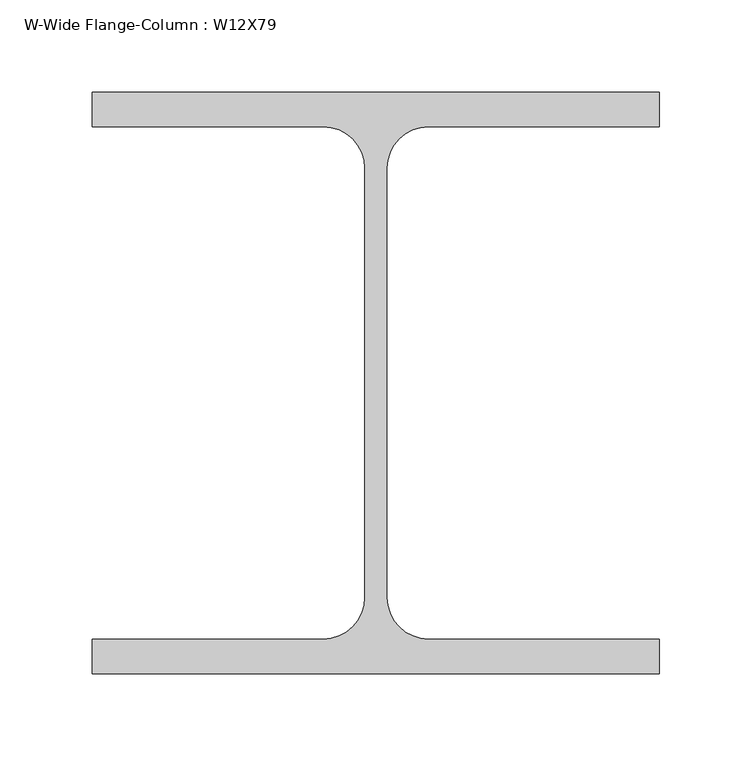
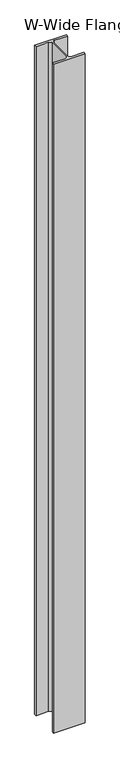
"""IFC4 building model written with IfcOpenShell, lengths in millimetres: column geometry, W-Wide Flange-Column : W12X79."""

from ifc_helpers import new_model, si_unit, point, frame, frame_2d, origin, place, context, project, spatial, polyline, circle_curve, trimmed, segment, composite_curve, outline, extrude, source, transform, mapped, element, save


def w_wide_flange_column_w12x79_acbb4a60(model_context):
    return source(origin(), model_context, "Body", "SweptSolid", [
        extrude(outline(composite_curve([segment(polyline([(153.67, 157.48), (153.67, 138.811), (28.575, 138.811)]), True, "CONTINUOUS"), segment(trimmed(circle_curve(frame_2d((28.575, 116.205)), 22.606), [point((28.575, 138.811))], [point((5.969, 116.205))], True, "CARTESIAN"), True, "CONTINUOUS"), segment(polyline([(5.969, 116.205), (5.969, -116.205)]), True, "CONTINUOUS"), segment(trimmed(circle_curve(frame_2d((28.575, -116.205)), 22.606), [point((5.969, -116.205))], [point((28.575, -138.811))], True, "CARTESIAN"), True, "CONTINUOUS"), segment(polyline([(28.575, -138.811), (153.67, -138.811), (153.67, -157.48), (-153.67, -157.48), (-153.67, -138.811), (-28.575, -138.811)]), True, "CONTINUOUS"), segment(trimmed(circle_curve(frame_2d((-28.575, -116.205)), 22.606), [point((-28.575, -138.811))], [point((-5.969, -116.205))], True, "CARTESIAN"), True, "CONTINUOUS"), segment(polyline([(-5.969, -116.205), (-5.969, 116.205)]), True, "CONTINUOUS"), segment(trimmed(circle_curve(frame_2d((-28.575, 116.205)), 22.606), [point((-5.969, 116.205))], [point((-28.575, 138.811))], True, "CARTESIAN"), True, "CONTINUOUS"), segment(polyline([(-28.575, 138.811), (-153.67, 138.811), (-153.67, 157.48), (153.67, 157.48)]), True, "CONTINUOUS")], self_intersect=False)), frame((0.0, 0.0, 8756.65), z_axis=(0.0, 0.0, 1.0), x_axis=(1.0, 0.0, 0.0)), (0.0, 0.0, 1.0), 6842.125),
    ])


if __name__ == "__main__":
    model = new_model("IFC4")
    model_context = context("Model", 3, world=origin())
    ifc_project = project(units=[si_unit("LENGTHUNIT", "METRE", prefix="MILLI")], contexts=[model_context])
    site = spatial("IfcSite", under=ifc_project)
    building = spatial("IfcBuilding", under=site)
    placement = place(None, origin())
    w_wide_flange_column_w12x79_shape = w_wide_flange_column_w12x79_acbb4a60(model_context)
    element("IfcColumn", 1, ObjectType="W-Wide Flange-Column : W12X79", at=placement, inside=building, context=model_context, shape_type="MappedRepresentation", body=[
        mapped(w_wide_flange_column_w12x79_shape, transform((0.0, 0.0, 0.0), x_axis=(1.0, 0.0, 0.0), y_axis=(0.0, 1.0, 0.0), z_axis=(0.0, 0.0, 1.0))),
    ])
    save(model, "model.ifc")

# Revit data of these elements
# Type "W-Wide Flange-Column : W12X79"
#   Assembly Code = "B10"
#   W = 79
#   bf = 1' - 0.1"
#   d = 1' - 0.4"
#   k = 0' - 1 5/8"
#   kr = 0' - 0.89"
#   tf = 0' - 0.735"
#   tw = 0' - 0.47"
#   A = 0.161111 SF
#   Structural Material [instance default] = Steel ASTM A992
# Element 1 (IfcColumn, "W-Wide Flange-Column : W12X79")
#   Materials on its faces: "Steel ASTM A992"
# Materials
#   "Steel ASTM A992": class "Metal", colour RGB 199 199 199, transparency 0, Description = "Structural steel 50ksi", Cost = 0
